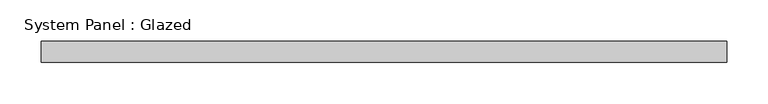
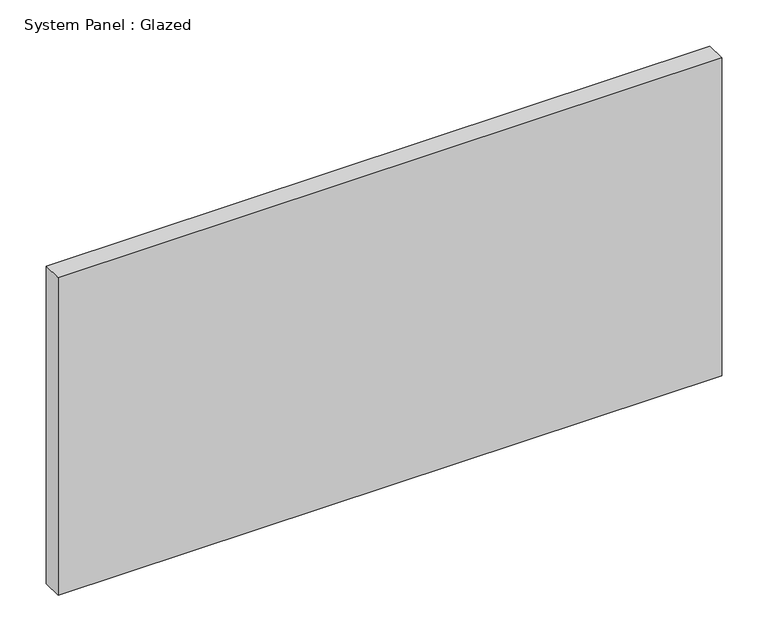
"""IFC4 building model written with IfcOpenShell, lengths in millimetres: plate geometry, System Panel : Glazed."""

import ifcopenshell
import ifcopenshell.guid

model = None  # the IFC model being written
_history = None  # IfcOwnerHistory: only IFC2X3 demands one
_inside = {}  # id of a spatial element -> (the spatial element, [elements in it])
_under = {}  # id of a project, library or spatial element -> (it, [spatial elements below it])
_declared = {}  # id of a project -> (the project, [libraries it declares])
_typed = {}  # id of a type object -> (the type object, [elements of that type])
_made_of = {}  # id of a material, layer set ... -> (it, [elements and type objects made of it])


def new_model(schema):
    """Start an empty IFC model of exactly this schema.

    Asked for "IFC4X3", IfcOpenShell would pick the latest addendum, in which some entities
    have other attributes; the version numbers below select the first issue.
    IFC2X3 requires an IfcOwnerHistory on every rooted entity: one is made here for all.
    """
    global model, _history
    if schema == "IFC4X3":
        model = ifcopenshell.file(schema_version=(4, 3, 0, 0))
    else:
        model = ifcopenshell.file(schema=schema)
    _inside.clear()
    _under.clear()
    _declared.clear()
    _typed.clear()
    _made_of.clear()
    _history = None
    if model.schema == "IFC2X3":
        org = make("IfcOrganization", Name="unknown")
        user = make(
            "IfcPersonAndOrganization",
            ThePerson=make("IfcPerson", FamilyName="unknown"),
            TheOrganization=org,
        )
        app = make(
            "IfcApplication",
            ApplicationDeveloper=org,
            Version="unknown",
            ApplicationFullName="unknown",
            ApplicationIdentifier="unknown",
        )
        _history = make(
            "IfcOwnerHistory",
            OwningUser=user,
            OwningApplication=app,
            ChangeAction="ADDED",
            CreationDate=0,
        )
    return model


def make(cls, **values):
    """One entity of the class cls with the attributes given. An attribute that is None is left unset."""
    return model.create_entity(
        cls, **{name: value for name, value in values.items() if value is not None}
    )


def rooted(cls, **values):
    """An entity with a GlobalId (a new one), such as an element, a storey or a relation."""
    return make(cls, GlobalId=ifcopenshell.guid.new(), OwnerHistory=_history, **values)


def si_unit(unit_type, name, prefix=None):
    """IfcSIUnit, for example si_unit("LENGTHUNIT", "METRE", prefix="MILLI")."""
    return make("IfcSIUnit", UnitType=unit_type, Prefix=prefix, Name=name)


def assignment(units):
    """IfcUnitAssignment: the units of a project."""
    return None if units is None else make("IfcUnitAssignment", Units=units)


def point(xyz):
    """IfcCartesianPoint."""
    return None if xyz is None else make("IfcCartesianPoint", Coordinates=xyz)


def direction(xyz):
    """IfcDirection."""
    return None if xyz is None else make("IfcDirection", DirectionRatios=xyz)


def frame(location, z_axis=None, x_axis=None):
    """IfcAxis2Placement3D, a coordinate frame: its origin and axes. An axis left out is left unset."""
    return make(
        "IfcAxis2Placement3D",
        Location=point(location),
        Axis=direction(z_axis),
        RefDirection=direction(x_axis),
    )


def origin():
    """The frame at (0, 0, 0) with its axes left unset."""
    return frame((0.0, 0.0, 0.0))


def origin_with_axes():
    """The frame at (0, 0, 0) with the z axis (0, 0, 1) and the x axis (1, 0, 0) written out."""
    return frame((0.0, 0.0, 0.0), z_axis=(0.0, 0.0, 1.0), x_axis=(1.0, 0.0, 0.0))


def place(relative_to, where):
    """IfcLocalPlacement: puts the frame where relative to a parent placement (None: the world)."""
    return make(
        "IfcLocalPlacement", PlacementRelTo=relative_to, RelativePlacement=where
    )


def context(
    kind, dimensions, precision=None, world=None, true_north=None, identifier=None
):
    """IfcGeometricRepresentationContext, for example the 3D "Model" context."""
    return make(
        "IfcGeometricRepresentationContext",
        ContextIdentifier=identifier,
        ContextType=kind,
        CoordinateSpaceDimension=dimensions,
        Precision=precision,
        WorldCoordinateSystem=world,
        TrueNorth=true_north,
    )


def project(units=None, contexts=None):
    """IfcProject with its units and contexts."""
    return rooted(
        "IfcProject",
        Name="project",
        RepresentationContexts=contexts,
        UnitsInContext=assignment(units),
    )


def spatial(cls, under=None, at=None, **own):
    """A site, building, storey or space (cls), placed at a placement, below another one or the project."""
    s = rooted(cls, ObjectPlacement=at, **own)
    if under is not None:
        _under.setdefault(under.id(), (under, []))[1].append(s)
    return s


def polyline(points):
    """IfcPolyline through the points."""
    return make("IfcPolyline", Points=[point(p) for p in points])


def outline(outer, holes=None, kind="AREA"):
    """IfcArbitraryClosedProfileDef: a profile drawn as a closed curve; with holes, ...WithVoids."""
    if holes is None:
        return make("IfcArbitraryClosedProfileDef", ProfileType=kind, OuterCurve=outer)
    return make(
        "IfcArbitraryProfileDefWithVoids",
        ProfileType=kind,
        OuterCurve=outer,
        InnerCurves=holes,
    )


def extrude(swept, where, along, depth):
    """IfcExtrudedAreaSolid: the profile swept, set in the frame where, extruded along a direction by depth."""
    return make(
        "IfcExtrudedAreaSolid",
        SweptArea=swept,
        Position=where,
        ExtrudedDirection=direction(along),
        Depth=depth,
    )


def shape(context_of_items, identifier, shape_type, items):
    """IfcShapeRepresentation: the items that make up one representation, for example the "Body"."""
    return make(
        "IfcShapeRepresentation",
        ContextOfItems=context_of_items,
        RepresentationIdentifier=identifier,
        RepresentationType=shape_type,
        Items=items,
    )


def source(mapping_origin, context_of_items, identifier, shape_type, items):
    """IfcRepresentationMap: a shape defined once, which mapped items show again and again."""
    return make(
        "IfcRepresentationMap",
        MappingOrigin=mapping_origin,
        MappedRepresentation=shape(context_of_items, identifier, shape_type, items),
    )


def transform(
    local_origin,
    x_axis=None,
    y_axis=None,
    z_axis=None,
    scale=None,
    scale2=None,
    scale3=None,
    uniform=True,
):
    """IfcCartesianTransformationOperator3D, or its non-uniform kind. x_axis, y_axis, z_axis: its Axis1, 2, 3."""
    if uniform:
        return make(
            "IfcCartesianTransformationOperator3D",
            Axis1=direction(x_axis),
            Axis2=direction(y_axis),
            LocalOrigin=point(local_origin),
            Scale=scale,
            Axis3=direction(z_axis),
        )
    return make(
        "IfcCartesianTransformationOperator3DnonUniform",
        Axis1=direction(x_axis),
        Axis2=direction(y_axis),
        LocalOrigin=point(local_origin),
        Scale=scale,
        Axis3=direction(z_axis),
        Scale2=scale2,
        Scale3=scale3,
    )


def mapped(mapping_source, mapping_target):
    """IfcMappedItem: shows the shape of a source again, moved by a transform."""
    return make(
        "IfcMappedItem", MappingSource=mapping_source, MappingTarget=mapping_target
    )


def made_of(thing, what):
    """Note that an element or type object is made of a material, layer set ...; save() writes the relation."""
    if what is not None:
        _made_of.setdefault(what.id(), (what, []))[1].append(thing)
    return thing


def element(
    cls,
    number,
    at=None,
    inside=None,
    cuts=None,
    type_object=None,
    material=None,
    context=None,
    identifier="Body",
    shape_type=None,
    held_by="IfcProductDefinitionShape",
    body=None,
    shapes=None,
    **own,
):
    """One element of the class cls, such as IfcWall. Its Tag is "e" and its number.

    at: its placement. inside: the storey or other place that contains it. cuts: it is an
    opening in that element (IfcRelVoidsElement). A single representation is given by context,
    identifier, shape_type and body (its items); several are given by shapes. held_by: the class
    of the entity that holds the representations. save() writes the other relations.
    """
    e = rooted(cls, Tag="e%d" % number, ObjectPlacement=at, **own)
    if body is not None:
        shapes = [shape(context, identifier, shape_type, body)]
    if shapes is not None:
        e.Representation = make(held_by, Representations=shapes)
    if inside is not None:
        _inside.setdefault(inside.id(), (inside, []))[1].append(e)
    if cuts is not None:
        rooted(
            "IfcRelVoidsElement", RelatingBuildingElement=cuts, RelatedOpeningElement=e
        )
    if type_object is not None:
        _typed.setdefault(type_object.id(), (type_object, []))[1].append(e)
    return made_of(e, material)


def aggregate(whole, parts):
    """IfcRelAggregates: a whole, such as a stair, and the parts it consists of."""
    return rooted("IfcRelAggregates", RelatingObject=whole, RelatedObjects=parts)


def save(model, path):
    """Write the relations noted so far, then the file.

    IfcRelAggregates (storeys below a building ...), IfcRelContainedInSpatialStructure (elements
    in a storey), IfcRelDefinesByType, IfcRelAssociatesMaterial and IfcRelDeclares: one each for
    every whole, place, type object, material and project.
    """
    for whole, parts in _under.values():
        aggregate(whole, parts)
    for where, things in _inside.values():
        rooted(
            "IfcRelContainedInSpatialStructure",
            RelatedElements=things,
            RelatingStructure=where,
        )
    for kind, things in _typed.values():
        rooted("IfcRelDefinesByType", RelatedObjects=things, RelatingType=kind)
    for what, things in _made_of.values():
        rooted("IfcRelAssociatesMaterial", RelatedObjects=things, RelatingMaterial=what)
    for by, libraries in _declared.values():
        rooted("IfcRelDeclares", RelatingContext=by, RelatedDefinitions=libraries)
    model.write(path)


def system_panel_glazed_9a7f91f8(model_context):
    return source(origin(), model_context, "Body", "SweptSolid", [
        extrude(outline(polyline([(414.0389939, 19.05), (-414.0389939, 19.05), (-414.0389939, 44.45), (414.0389939, 44.45), (414.0389939, 19.05)])), origin_with_axes(), (0.0, 0.0, 1.0), 419.1),
    ])


if __name__ == "__main__":
    model = new_model("IFC4")
    model_context = context("Model", 3, world=origin())
    ifc_project = project(units=[si_unit("LENGTHUNIT", "METRE", prefix="MILLI")], contexts=[model_context])
    site = spatial("IfcSite", under=ifc_project)
    building = spatial("IfcBuilding", under=site)
    placement = place(None, origin())
    system_panel_glazed_shape = system_panel_glazed_9a7f91f8(model_context)
    element("IfcPlate", 1, ObjectType="System Panel : Glazed", at=placement, inside=building, context=model_context, shape_type="MappedRepresentation", body=[
        mapped(system_panel_glazed_shape, transform((0.0, 0.0, 0.0), x_axis=(1.0, 0.0, 0.0), y_axis=(0.0, 1.0, 0.0), z_axis=(0.0, 0.0, 1.0))),
    ])
    save(model, "model.ifc")

# Revit data of these elements
# Type "System Panel : Glazed"
#   Construction Type Id = "GSP4R"
#   Analytic Construction = "1/8 in Pilkington single glazing"
#   Visual Light Transmittance = 0.9
#   Solar Heat Gain Coefficient = 0.86
#   Heat Transfer Coefficient (U) = 1.18115 BTU/(h·ft²·°F)
#   Define Thermal Properties by = 1
# Element 1 (IfcPlate, "System Panel : Glazed")
#   Materials on its faces: "Glass"
# Materials
#   "Glass": class "Glass", colour RGB 0 128 192, transparency 0.75, Description = "Soda Lime Glass", Cost = 0
